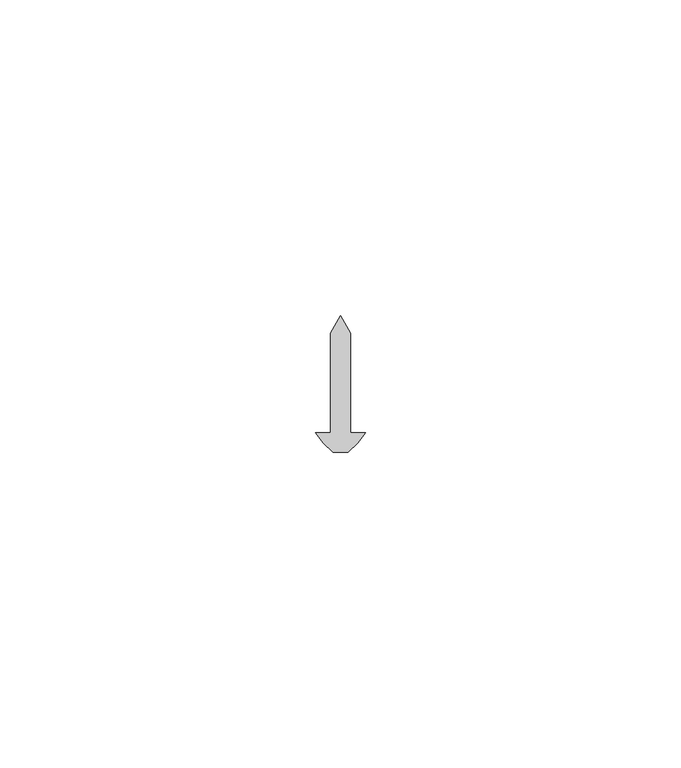
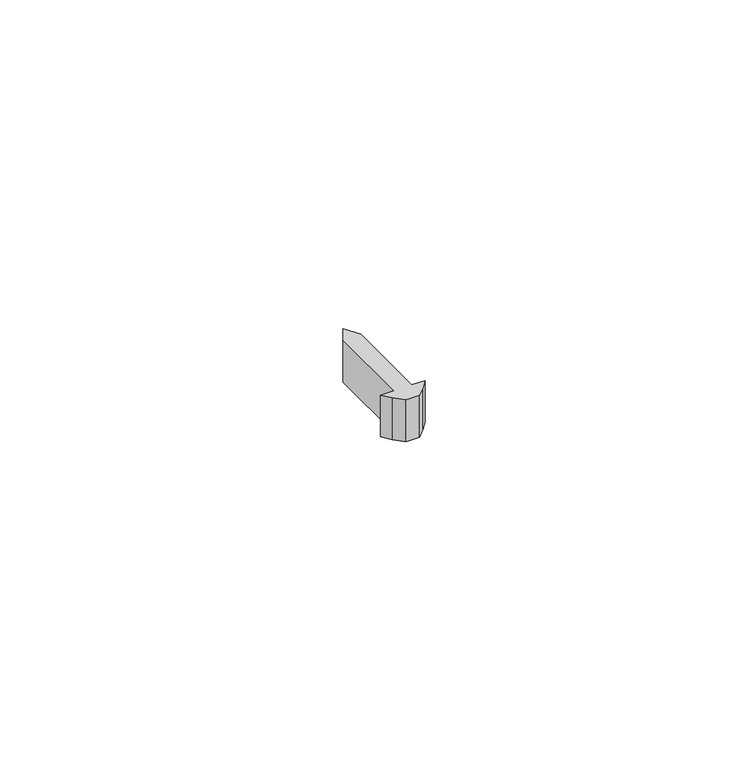
"""IFC4 building model written with IfcOpenShell, lengths in millimetres: proxy geometry, Generic Models 7:Generic Models 1:3:Generic Models 1:3 : Generic Models 7:Generic Models 1:305549:3:Generic Models 1:3:Generic Models 1:3 : Generic Models 7:Generic Models 1:305549:3 : Generic Models 7:Generic Models 1:3:Generic Models 1:3 : Generic Models 7:Generic Models 1:305549:301244:24 : Generic Models 7:Generic Models 1:3:Generic Models 1:3 : Generic Models 7:Generic Models 1:305549:3:Generic Models 1:3:Generic Models 1:3 : Generic Models 7:Generic Models 1:305549:3 : Generic Models 7:Generic Models 1:3:Generic Models 1:3 : Generic Models 7:Generic Models 1:305549:301244:308848."""

from ifc_helpers import new_model, si_unit, frame, origin, place, context, project, spatial, polyline, outline, extrude, source, transform, mapped, element, save


def generic_models_cc22baa6(model_context):
    return source(origin(), model_context, "Body", "SweptSolid", [
        extrude(outline(polyline([(560367.2492239, -579084.8288841), (560369.6304739, -579084.8288841), (560368.4122783, -579086.3559421), (560366.8603881, -579087.9078323), (560364.4630596, -579087.9078323), (560362.9111694, -579086.3559421), (560361.6929739, -579084.8288841), (560364.0742239, -579084.8288841), (560364.0742239, -579069.0196286), (560365.6617239, -579066.2699979), (560367.2492239, -579069.0196286), (560367.2492239, -579084.8288841)])), frame((0.0, 0.0, 4907.75625), z_axis=(0.0, 0.0, 1.0), x_axis=(1.0, 0.0, 0.0)), (0.0, 0.0, 1.0), 7.9375),
    ])


if __name__ == "__main__":
    model = new_model("IFC4")
    model_context = context("Model", 3, world=origin())
    ifc_project = project(units=[si_unit("LENGTHUNIT", "METRE", prefix="MILLI")], contexts=[model_context])
    site = spatial("IfcSite", under=ifc_project)
    building = spatial("IfcBuilding", under=site)
    placement = place(None, origin())
    generic_models_shape = generic_models_cc22baa6(model_context)
    element("IfcBuildingElementProxy", 1, Name="Generic Models 7:Generic Models 1:3:Generic Models 1:3 : Generic Models 7:Generic Models 1:305549:3:Generic Models 1:3:Generic Models 1:3 : Generic Models 7:Generic Models 1:305549:3 : Generic Models 7:Generic Models 1:3:Generic Models 1:3 : Generic Models 7:Generic Models 1:305549:301244:24 : Generic Models 7:Generic Models 1:3:Generic Models 1:3 : Generic Models 7:Generic Models 1:305549:3:Generic Models 1:3:Generic Models 1:3 : Generic Models 7:Generic Models 1:305549:3 : Generic Models 7:Generic Models 1:3:Generic Models 1:3 : Generic Models 7:Generic Models 1:305549:301244:308848", ObjectType="Generic Models 7:Generic Models 1:3:Generic Models 1:3 : Generic Models 7:Generic Models 1:305549:3:Generic Models 1:3:Generic Models 1:3 : Generic Models 7:Generic Models 1:305549:3 : Generic Models 7:Generic Models 1:3:Generic Models 1:3 : Generic Models 7:Generic Models 1:305549:301244:24 : Generic Models 7:Generic Models 1:3:Generic Models 1:3 : Generic Models 7:Generic Models 1:305549:3:Generic Models 1:3:Generic Models 1:3 : Generic Models 7:Generic Models 1:305549:3 : Generic Models 7:Generic Models 1:3:Generic Models 1:3 : Generic Models 7:Generic Models 1:305549:301244:308848", at=placement, inside=building, context=model_context, shape_type="MappedRepresentation", body=[
        mapped(generic_models_shape, transform((0.0, 0.0, 0.0), x_axis=(1.0, 0.0, 0.0), y_axis=(0.0, 1.0, 0.0), z_axis=(0.0, 0.0, 1.0))),
    ])
    save(model, "model.ifc")

# Revit data of these elements
# Type "Generic Models 7:Generic Models 1:3:Generic Models 1:3 : Generic Models 7:Generic Models 1:305549:3:Generic Models 1:3:Generic Models 1:3 : Generic Models 7:Generic Models 1:305549:3 : Generic Models 7:Generic Models 1:3:Generic Models 1:3 : Generic Models 7:Generic Models 1:305549:301244:24 : Generic Models 7:Generic Models 1:3:Generic Models 1:3 : Generic Models 7:Generic Models 1:305549:3:Generic Models 1:3:Generic Models 1:3 : Generic Models 7:Generic Models 1:305549:3 : Generic Models 7:Generic Models 1:3:Generic Models 1:3 : Generic Models 7:Generic Models 1:305549:301244:308848"
#   NameOverride = "Generic Models 7:Generic Models 1:3:Generic Models 1:3 : Generic Models 7:Generic Models 1:305549:3:Generic Models 1:3:Generic Models 1:3 : Generic Models 7:Generic Models 1:305549:3 : Generic Models 7:Generic Models 1:3:Generic Models 1:3 : Generic Models 7:Generic Models 1:305549:301244:308848"
#   ObjectTypeOverride = "Generic Models 1:3:Generic Models 1:3 : Generic Models 7:Generic Models 1:305549:3 : Generic Models 7:Generic Models 1:3:Generic Models 1:3 : Generic Models 7:Generic Models 1:305549:301244"
#   Reference = "Generic Models 1"
#   Tag = "308848"
# Element 1 (IfcBuildingElementProxy, "Generic Models 7:Generic Models 1:3:Generic Models 1:3 : Generic Models 7:Generic Models 1:305549:3:Generic Models 1:3:Generic Models 1:3 : Generic Models 7:Generic Models 1:305549:3 : Generic Models 7:Generic Models 1:3:Generic Models 1:3 : Generic Models 7:Generic Models 1:305549:301244:24 : Generic Models 7:Generic Models 1:3:Generic Models 1:3 : Generic Models 7:Generic Models 1:305549:3:Generic Models 1:3:Generic Models 1:3 : Generic Models 7:Generic Models 1:305549:3 : Generic Models 7:Generic Models 1:3:Generic Models 1:3 : Generic Models 7:Generic Models 1:305549:301244:308848")
#   Materials on its faces: "FASTENERS (T.B.D)"
# Materials
#   "FASTENERS (T.B.D)": class "Generic", colour RGB 120 120 120, transparency 0, Cost = 0
